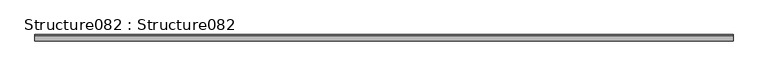
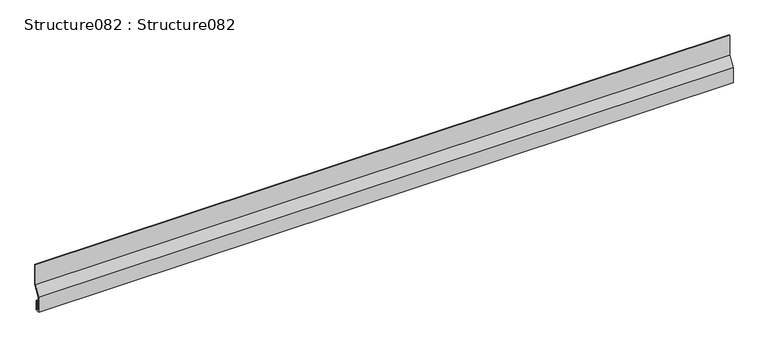
"""IFC4 building model written with IfcOpenShell, lengths in millimetres: proxy geometry, Structure082 : Structure082."""

from ifc_helpers import new_model, si_unit, frame, origin, place, context, project, spatial, polyline, outline, extrude, source, transform, mapped, element, save


def structure082_structure082_972cd440(model_context):
    return source(origin(), model_context, "Body", "SweptSolid", [
        extrude(outline(polyline([(4455.945844, 41622.6975349), (4440.1001444, 41593.7180987), (4440.1001444, 41552.3384125), (4447.7201388, 41552.3384125), (4447.7201388, 41578.6076619), (4450.2601388, 41578.6076619), (4450.2601388, 41549.8080335), (4437.5601444, 41549.8080335), (4437.5601444, 41594.3671762), (4453.405844, 41623.3466124), (4453.405844, 41683.7015982), (4455.945844, 41683.7015982), (4455.945844, 41622.6975349)])), frame((255.0171875, 0.0, 0.0), z_axis=(1.0, 0.0, 0.0), x_axis=(0.0, 1.0, 0.0)), (0.0, 0.0, 1.0), 1999.85),
    ])


if __name__ == "__main__":
    model = new_model("IFC4")
    model_context = context("Model", 3, world=origin())
    ifc_project = project(units=[si_unit("LENGTHUNIT", "METRE", prefix="MILLI")], contexts=[model_context])
    site = spatial("IfcSite", under=ifc_project)
    building = spatial("IfcBuilding", under=site)
    placement = place(None, origin())
    structure082_structure082_shape = structure082_structure082_972cd440(model_context)
    element("IfcBuildingElementProxy", 1, Name="Structure082 : Structure082", ObjectType="Structure082 : Structure082", at=placement, inside=building, context=model_context, shape_type="MappedRepresentation", body=[
        mapped(structure082_structure082_shape, transform((0.0, 0.0, 0.0), x_axis=(1.0, 0.0, 0.0), y_axis=(0.0, 1.0, 0.0), z_axis=(0.0, 0.0, 1.0))),
    ])
    save(model, "model.ifc")

# Revit data of these elements
# Type "Structure082 : Structure082"
#   NameOverride = "Structure082"
# Element 1 (IfcBuildingElementProxy, "Structure082 : Structure082")
#   Materials on its faces: "COUNTER FLASHING"
# Materials
#   "COUNTER FLASHING": class "Unassigned", colour RGB 128 128 128, transparency 0
